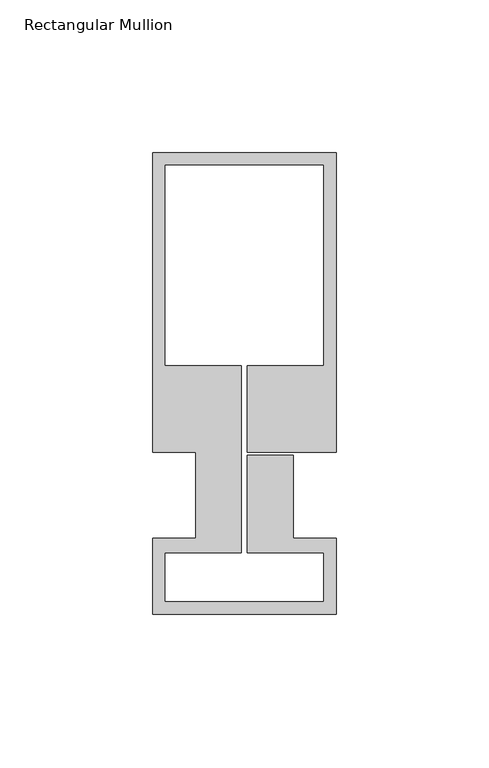
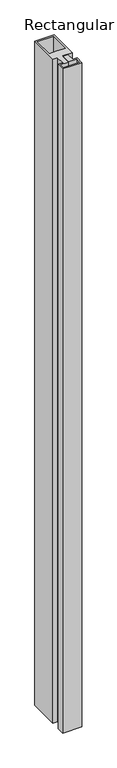
"""IFC4 building model written with IfcOpenShell, lengths in millimetres: member geometry, Rectangular Mullion : Schueco_FWS-60-HI_Mull_CovCap-20mm_Mull-85mm."""

from ifc_helpers import new_model, si_unit, frame, origin, place, context, project, spatial, polyline, outline, extrude, source, transform, mapped, element, save


def rectangular_mullion_792441dc(model_context):
    return source(origin(), model_context, "Body", "SweptSolid", [
        extrude(outline(polyline([(-60.0, 126.0), (0.0, 126.0), (0.0, 28.0), (-29.0, 28.0), (-29.0, 56.3), (-4.0, 56.3), (-4.0, 122.0), (-56.0, 122.0), (-56.0, 56.3), (-31.0, 56.3), (-31.0, -5.0), (-56.0, -5.0), (-56.0, -21.0), (-4.0, -21.0), (-4.0, -5.0), (-29.0, -5.0), (-29.0, 27.0), (-14.0, 27.0), (-14.0, -0.1), (0.0, -0.1), (0.0, -25.0), (-60.0, -25.0), (-60.0, -0.1), (-46.0, -0.1), (-46.0, 28.0), (-60.0, 28.0), (-60.0, 126.0)])), frame((0.0, 0.0, -2200.0), z_axis=(0.0, 0.0, 1.0), x_axis=(1.0, 0.0, 0.0)), (0.0, 0.0, 1.0), 2200.0),
    ])


if __name__ == "__main__":
    model = new_model("IFC4")
    model_context = context("Model", 3, world=origin())
    ifc_project = project(units=[si_unit("LENGTHUNIT", "METRE", prefix="MILLI")], contexts=[model_context])
    site = spatial("IfcSite", under=ifc_project)
    building = spatial("IfcBuilding", under=site)
    placement = place(None, origin())
    rectangular_mullion_shape = rectangular_mullion_792441dc(model_context)
    element("IfcMember", 1, ObjectType="Rectangular Mullion : Schueco_FWS-60-HI_Mull_CovCap-20mm_Mull-85mm", at=placement, inside=building, context=model_context, shape_type="MappedRepresentation", body=[
        mapped(rectangular_mullion_shape, transform((0.0, 0.0, 0.0), x_axis=(1.0, 0.0, 0.0), y_axis=(0.0, 1.0, 0.0), z_axis=(0.0, 0.0, 1.0))),
    ])
    save(model, "model.ifc")

# Revit data of these elements
# Type "Rectangular Mullion : Schueco_FWS-60-HI_Mull_CovCap-20mm_Mull-85mm"
#   Model = "FWS 60.HI"
#   Manufacturer = "Schueco International KG"
#   Type Comments = "Mullion"
#   Schueco thermal insulation standard = "Highly thermally insulated"
#   Burglar resistance = "RC 3"
#   Thermal insulation = "to 0.90 W/(m²K)"
#   built-in parameter 1007322 = 0.495407 (stored number, unit not read)
#   built-in parameter 1007321 = 0.0524934 (stored number, unit not read)
#   built-in parameter 1007320 = 0.0524934 (stored number, unit not read)
# Element 1 (IfcMember, "Rectangular Mullion : Schueco_FWS-60-HI_Mull_CovCap-20mm_Mull-85mm")
#   Materials on its faces: "Alu"
# Materials
#   "Alu": class "Glas", colour RGB 140 140 140, transparency 0
